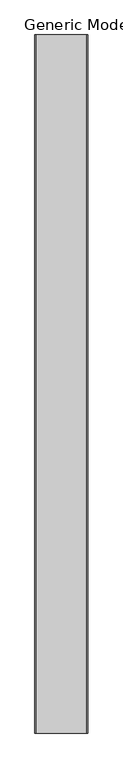
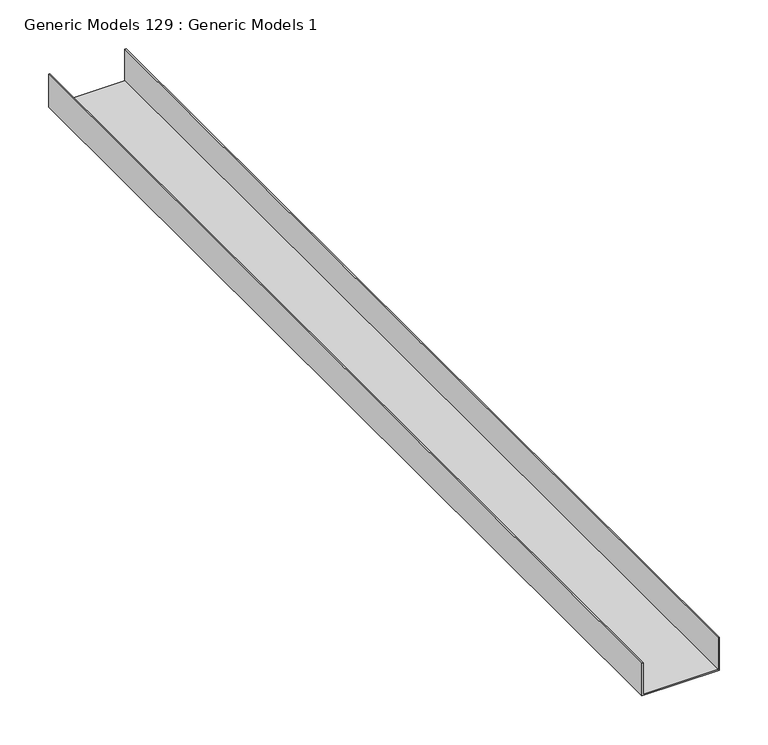
"""IFC4 building model written with IfcOpenShell, lengths in millimetres: proxy geometry, Generic Models 129 : Generic Models 1."""

from ifc_helpers import new_model, si_unit, frame, origin, place, context, project, spatial, polyline, outline, extrude, source, transform, mapped, element, save


def generic_models_129_generic_models_1_ee561edf(model_context):
    return source(origin(), model_context, "Body", "SweptSolid", [
        extrude(outline(polyline([(0.0, 50793.65), (0.0, 50885.725), (41.275, 50885.725), (41.275, 50884.1375), (1.5875, 50884.1375), (1.5875, 50795.2375), (41.275, 50795.2375), (41.275, 50793.65), (0.0, 50793.65)])), frame((0.0, 0.0, 0.0), z_axis=(0.0, 1.0, 0.0), x_axis=(0.0, 0.0, 1.0)), (0.0, 0.0, 1.0), 1219.2),
    ])


if __name__ == "__main__":
    model = new_model("IFC4")
    model_context = context("Model", 3, world=origin())
    ifc_project = project(units=[si_unit("LENGTHUNIT", "METRE", prefix="MILLI")], contexts=[model_context])
    site = spatial("IfcSite", under=ifc_project)
    building = spatial("IfcBuilding", under=site)
    placement = place(None, origin())
    generic_models_129_generic_models_1_shape = generic_models_129_generic_models_1_ee561edf(model_context)
    element("IfcBuildingElementProxy", 1, Name="Generic Models 129 : Generic Models 1", ObjectType="Generic Models 129 : Generic Models 1", at=placement, inside=building, context=model_context, shape_type="MappedRepresentation", body=[
        mapped(generic_models_129_generic_models_1_shape, transform((0.0, 0.0, 0.0), x_axis=(1.0, 0.0, 0.0), y_axis=(0.0, 1.0, 0.0), z_axis=(0.0, 0.0, 1.0))),
    ])
    save(model, "model.ifc")

# Revit data of these elements
# Element 1 (IfcBuildingElementProxy, "Generic Models 129 : Generic Models 1")
#   Materials on its faces: "METAL RUNNER ANCHORED TO STRUCTURE"
# Materials
#   "METAL RUNNER ANCHORED TO STRUCTURE": class "Unassigned", colour RGB 210 209 208, transparency 0, Keynote = "M05121300.02", Cost = 0
